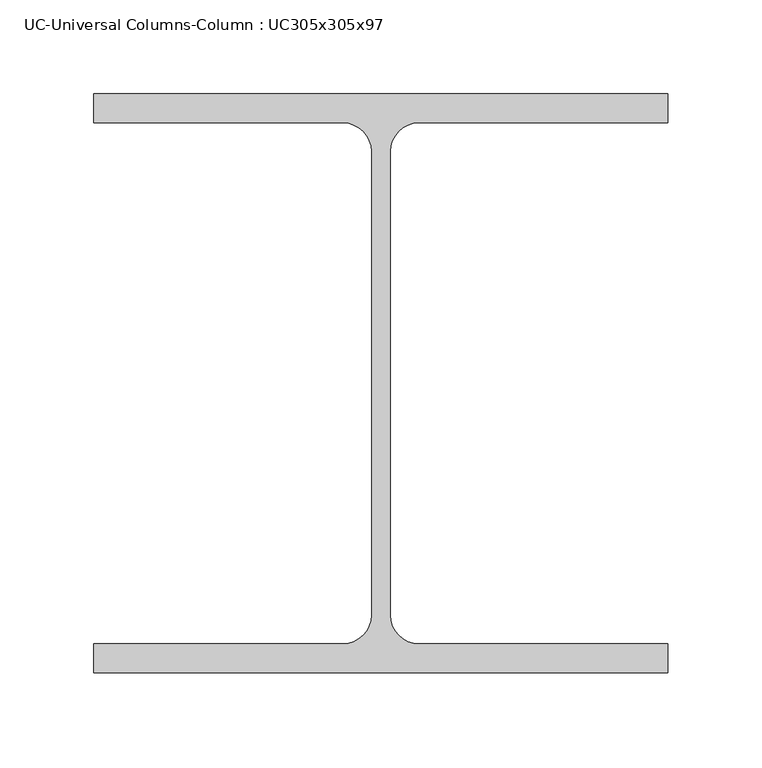
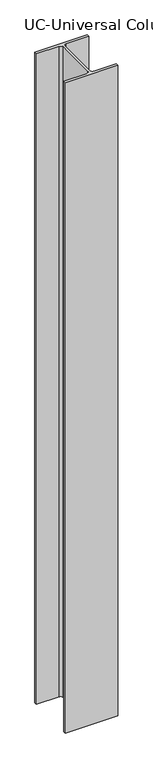
"""IFC4 building model written with IfcOpenShell, lengths in millimetres: column geometry, UC-Universal Columns-Column : UC305x305x97."""

from ifc_helpers import new_model, si_unit, point, frame_2d, origin, origin_with_axes, place, context, project, spatial, polyline, circle_curve, trimmed, segment, composite_curve, outline, extrude, source, transform, mapped, element, save


def uc_universal_columns_column_uc305x305x97_7d345059(model_context):
    return source(origin(), model_context, "Body", "SweptSolid", [
        extrude(outline(composite_curve([segment(polyline([(152.65, -153.95), (-152.65, -153.95), (-152.65, -138.55), (-20.15, -138.55)]), True, "CONTINUOUS"), segment(trimmed(circle_curve(frame_2d((-20.15, -123.35)), 15.2), [point((-20.15, -138.55))], [point((-4.95, -123.35))], True, "CARTESIAN"), True, "CONTINUOUS"), segment(polyline([(-4.95, -123.35), (-4.95, 123.35)]), True, "CONTINUOUS"), segment(trimmed(circle_curve(frame_2d((-20.15, 123.35)), 15.2), [point((-4.95, 123.35))], [point((-20.15, 138.55))], True, "CARTESIAN"), True, "CONTINUOUS"), segment(polyline([(-20.15, 138.55), (-152.65, 138.55), (-152.65, 153.95), (152.65, 153.95), (152.65, 138.55), (20.15, 138.55)]), True, "CONTINUOUS"), segment(trimmed(circle_curve(frame_2d((20.15, 123.35)), 15.2), [point((20.15, 138.55))], [point((4.95, 123.35))], True, "CARTESIAN"), True, "CONTINUOUS"), segment(polyline([(4.95, 123.35), (4.95, -123.35)]), True, "CONTINUOUS"), segment(trimmed(circle_curve(frame_2d((20.15, -123.35)), 15.2), [point((4.95, -123.35))], [point((20.15, -138.55))], True, "CARTESIAN"), True, "CONTINUOUS"), segment(polyline([(20.15, -138.55), (152.65, -138.55), (152.65, -153.95)]), True, "CONTINUOUS")], self_intersect=False)), origin_with_axes(), (0.0, 0.0, 1.0), 4000.0),
    ])


if __name__ == "__main__":
    model = new_model("IFC4")
    model_context = context("Model", 3, world=origin())
    ifc_project = project(units=[si_unit("LENGTHUNIT", "METRE", prefix="MILLI")], contexts=[model_context])
    site = spatial("IfcSite", under=ifc_project)
    building = spatial("IfcBuilding", under=site)
    placement = place(None, origin())
    uc_universal_columns_column_uc305x305x97_shape = uc_universal_columns_column_uc305x305x97_7d345059(model_context)
    element("IfcColumn", 1, ObjectType="UC-Universal Columns-Column : UC305x305x97", at=placement, inside=building, context=model_context, shape_type="MappedRepresentation", body=[
        mapped(uc_universal_columns_column_uc305x305x97_shape, transform((0.0, 0.0, 0.0), x_axis=(1.0, 0.0, 0.0), y_axis=(0.0, 1.0, 0.0), z_axis=(0.0, 0.0, 1.0))),
    ])
    save(model, "model.ifc")

# Revit data of these elements
# Type "UC-Universal Columns-Column : UC305x305x97"
#   Section Name Key = "UC305x305x97"
#   Width = 30.53 cm
#   Web Thickness = 0.99 cm
#   Web Fillet = 1.52 cm
#   Warping Constant = 1560000.0 cm⁶
#   Torsional Moment of Inertia = 91.20 cm⁴
#   Section Area = 123.0 cm²
#   Plastic Modulus weak axis = 726.0 cm³
#   Plastic Modulus strong axis = 1592.0 cm³
#   Nominal Weight = 96.8996 kgf/m
#   Moment of Inertia weak axis = 7308.00 cm⁴
#   Moment of Inertia strong axis = 22249.00 cm⁴
#   Height = 30.79 cm
#   Flange Thickness = 1.54 cm
#   Elastic Modulus weak axis = 479.0 cm³
#   Elastic Modulus strong axis = 1445.0 cm³
#   Centroid Vertical = 15.395 cm
#   Centroid Horizontal = 15.265 cm
#   Bolt Spacing = 14.0 cm
#   Structural Material [instance default] = Metal - Steel 43-275
#   Type Comments = ""
#   Assembly Code = ""
# Element 1 (IfcColumn, "UC-Universal Columns-Column : UC305x305x97")
#   Materials on its faces: "Metal - Steel 43-275"
# Materials
#   "Metal - Steel 43-275": class "Metal", colour RGB 247 247 247, transparency 0, Cost = 0
